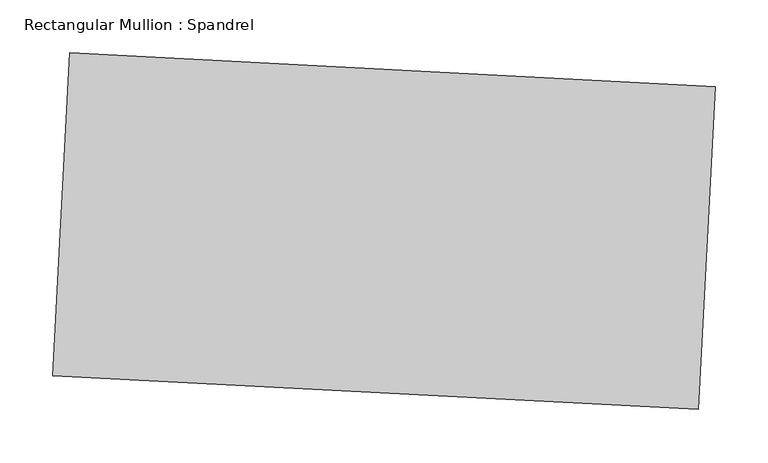
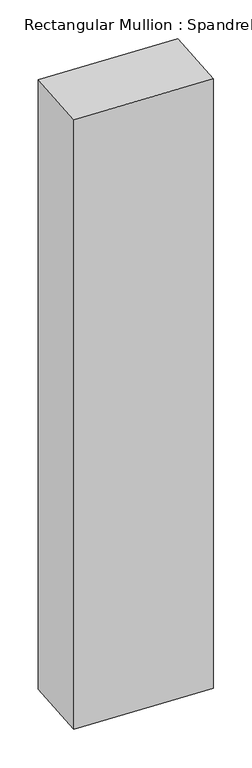
"""IFC4 building model written with IfcOpenShell, lengths in millimetres: member geometry, Rectangular Mullion : Spandrel."""

from ifc_helpers import new_model, si_unit, frame, origin, place, context, project, spatial, polyline, outline, extrude, source, transform, mapped, element, save


def rectangular_mullion_spandrel_ef47994c(model_context):
    return source(origin(), model_context, "Body", "SweptSolid", [
        extrude(outline(polyline([(7.5582819, 136.2391416), (-8.3937175, -168.1431406), (-617.1582819, -136.2391416), (-601.2062825, 168.1431406), (7.5582819, 136.2391416)])), frame((0.0, 0.0, -2900.7036942), z_axis=(0.0, 0.0, 1.0), x_axis=(1.0, 0.0, 0.0)), (0.0, 0.0, 1.0), 2900.7036942),
    ])


if __name__ == "__main__":
    model = new_model("IFC4")
    model_context = context("Model", 3, world=origin())
    ifc_project = project(units=[si_unit("LENGTHUNIT", "METRE", prefix="MILLI")], contexts=[model_context])
    site = spatial("IfcSite", under=ifc_project)
    building = spatial("IfcBuilding", under=site)
    placement = place(None, origin())
    rectangular_mullion_spandrel_shape = rectangular_mullion_spandrel_ef47994c(model_context)
    element("IfcMember", 1, ObjectType="Rectangular Mullion : Spandrel", at=placement, inside=building, context=model_context, shape_type="MappedRepresentation", body=[
        mapped(rectangular_mullion_spandrel_shape, transform((0.0, 0.0, 0.0), x_axis=(1.0, 0.0, 0.0), y_axis=(0.0, 1.0, 0.0), z_axis=(0.0, 0.0, 1.0))),
    ])
    save(model, "model.ifc")

# Revit data of these elements
# Type "Rectangular Mullion : Spandrel"
#   built-in parameter 1007304 = 1 (stored number, unit not read)
#   built-in parameter 1007301 = 1 (stored number, unit not read)
#   built-in parameter 1007300 = 1 (stored number, unit not read)
# Element 1 (IfcMember, "Rectangular Mullion : Spandrel")
#   Materials on its faces: "Aluminum"
# Materials
#   "Aluminum": class "Metal", colour RGB 247 247 247, transparency 0, Description = "Aluminum 6061", Cost = 0
